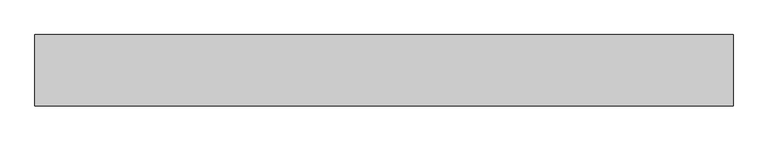
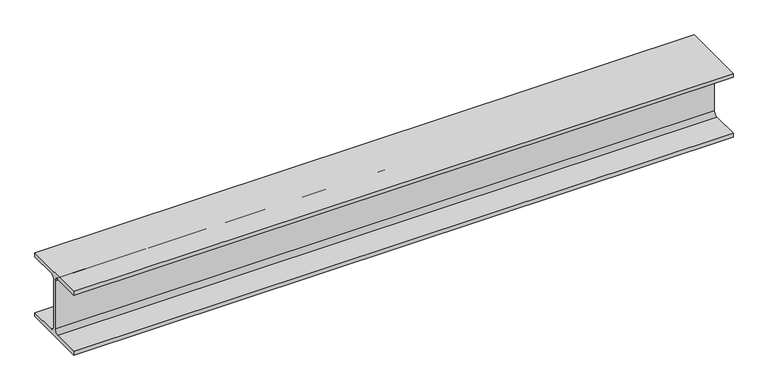
"""IFC4 building model written with IfcOpenShell, lengths in millimetres: beam geometry, 0912_Steel Framing_H-KSD3502 : H_SB_ASB_H-200x200x8x12."""

import ifcopenshell
import ifcopenshell.guid

model = None  # the IFC model being written
_history = None  # IfcOwnerHistory: only IFC2X3 demands one
_inside = {}  # id of a spatial element -> (the spatial element, [elements in it])
_under = {}  # id of a project, library or spatial element -> (it, [spatial elements below it])
_declared = {}  # id of a project -> (the project, [libraries it declares])
_typed = {}  # id of a type object -> (the type object, [elements of that type])
_made_of = {}  # id of a material, layer set ... -> (it, [elements and type objects made of it])


def new_model(schema):
    """Start an empty IFC model of exactly this schema.

    Asked for "IFC4X3", IfcOpenShell would pick the latest addendum, in which some entities
    have other attributes; the version numbers below select the first issue.
    IFC2X3 requires an IfcOwnerHistory on every rooted entity: one is made here for all.
    """
    global model, _history
    if schema == "IFC4X3":
        model = ifcopenshell.file(schema_version=(4, 3, 0, 0))
    else:
        model = ifcopenshell.file(schema=schema)
    _inside.clear()
    _under.clear()
    _declared.clear()
    _typed.clear()
    _made_of.clear()
    _history = None
    if model.schema == "IFC2X3":
        org = make("IfcOrganization", Name="unknown")
        user = make(
            "IfcPersonAndOrganization",
            ThePerson=make("IfcPerson", FamilyName="unknown"),
            TheOrganization=org,
        )
        app = make(
            "IfcApplication",
            ApplicationDeveloper=org,
            Version="unknown",
            ApplicationFullName="unknown",
            ApplicationIdentifier="unknown",
        )
        _history = make(
            "IfcOwnerHistory",
            OwningUser=user,
            OwningApplication=app,
            ChangeAction="ADDED",
            CreationDate=0,
        )
    return model


def make(cls, **values):
    """One entity of the class cls with the attributes given. An attribute that is None is left unset."""
    return model.create_entity(
        cls, **{name: value for name, value in values.items() if value is not None}
    )


def rooted(cls, **values):
    """An entity with a GlobalId (a new one), such as an element, a storey or a relation."""
    return make(cls, GlobalId=ifcopenshell.guid.new(), OwnerHistory=_history, **values)


def si_unit(unit_type, name, prefix=None):
    """IfcSIUnit, for example si_unit("LENGTHUNIT", "METRE", prefix="MILLI")."""
    return make("IfcSIUnit", UnitType=unit_type, Prefix=prefix, Name=name)


def assignment(units):
    """IfcUnitAssignment: the units of a project."""
    return None if units is None else make("IfcUnitAssignment", Units=units)


def point(xyz):
    """IfcCartesianPoint."""
    return None if xyz is None else make("IfcCartesianPoint", Coordinates=xyz)


def direction(xyz):
    """IfcDirection."""
    return None if xyz is None else make("IfcDirection", DirectionRatios=xyz)


def frame(location, z_axis=None, x_axis=None):
    """IfcAxis2Placement3D, a coordinate frame: its origin and axes. An axis left out is left unset."""
    return make(
        "IfcAxis2Placement3D",
        Location=point(location),
        Axis=direction(z_axis),
        RefDirection=direction(x_axis),
    )


def frame_2d(location, x_axis=None):
    """IfcAxis2Placement2D, a coordinate frame in the plane: its origin and x axis."""
    return make(
        "IfcAxis2Placement2D", Location=point(location), RefDirection=direction(x_axis)
    )


def origin():
    """The frame at (0, 0, 0) with its axes left unset."""
    return frame((0.0, 0.0, 0.0))


def place(relative_to, where):
    """IfcLocalPlacement: puts the frame where relative to a parent placement (None: the world)."""
    return make(
        "IfcLocalPlacement", PlacementRelTo=relative_to, RelativePlacement=where
    )


def context(
    kind, dimensions, precision=None, world=None, true_north=None, identifier=None
):
    """IfcGeometricRepresentationContext, for example the 3D "Model" context."""
    return make(
        "IfcGeometricRepresentationContext",
        ContextIdentifier=identifier,
        ContextType=kind,
        CoordinateSpaceDimension=dimensions,
        Precision=precision,
        WorldCoordinateSystem=world,
        TrueNorth=true_north,
    )


def project(units=None, contexts=None):
    """IfcProject with its units and contexts."""
    return rooted(
        "IfcProject",
        Name="project",
        RepresentationContexts=contexts,
        UnitsInContext=assignment(units),
    )


def spatial(cls, under=None, at=None, **own):
    """A site, building, storey or space (cls), placed at a placement, below another one or the project."""
    s = rooted(cls, ObjectPlacement=at, **own)
    if under is not None:
        _under.setdefault(under.id(), (under, []))[1].append(s)
    return s


def polyline(points):
    """IfcPolyline through the points."""
    return make("IfcPolyline", Points=[point(p) for p in points])


def circle_curve(where, radius):
    """IfcCircle in the frame where."""
    return make("IfcCircle", Position=where, Radius=radius)


def trimmed(basis, trim1, trim2, sense, master):
    """IfcTrimmedCurve: the piece of a basis curve between two trims."""
    return make(
        "IfcTrimmedCurve",
        BasisCurve=basis,
        Trim1=trim1,
        Trim2=trim2,
        SenseAgreement=sense,
        MasterRepresentation=master,
    )


def segment(curve, same_sense, transition):
    """IfcCompositeCurveSegment."""
    return make(
        "IfcCompositeCurveSegment",
        Transition=transition,
        SameSense=same_sense,
        ParentCurve=curve,
    )


def composite_curve(segments, self_intersect=None):
    """IfcCompositeCurve: segments joined end to end."""
    return make("IfcCompositeCurve", Segments=segments, SelfIntersect=self_intersect)


def outline(outer, holes=None, kind="AREA"):
    """IfcArbitraryClosedProfileDef: a profile drawn as a closed curve; with holes, ...WithVoids."""
    if holes is None:
        return make("IfcArbitraryClosedProfileDef", ProfileType=kind, OuterCurve=outer)
    return make(
        "IfcArbitraryProfileDefWithVoids",
        ProfileType=kind,
        OuterCurve=outer,
        InnerCurves=holes,
    )


def extrude(swept, where, along, depth):
    """IfcExtrudedAreaSolid: the profile swept, set in the frame where, extruded along a direction by depth."""
    return make(
        "IfcExtrudedAreaSolid",
        SweptArea=swept,
        Position=where,
        ExtrudedDirection=direction(along),
        Depth=depth,
    )


def shape(context_of_items, identifier, shape_type, items):
    """IfcShapeRepresentation: the items that make up one representation, for example the "Body"."""
    return make(
        "IfcShapeRepresentation",
        ContextOfItems=context_of_items,
        RepresentationIdentifier=identifier,
        RepresentationType=shape_type,
        Items=items,
    )


def source(mapping_origin, context_of_items, identifier, shape_type, items):
    """IfcRepresentationMap: a shape defined once, which mapped items show again and again."""
    return make(
        "IfcRepresentationMap",
        MappingOrigin=mapping_origin,
        MappedRepresentation=shape(context_of_items, identifier, shape_type, items),
    )


def transform(
    local_origin,
    x_axis=None,
    y_axis=None,
    z_axis=None,
    scale=None,
    scale2=None,
    scale3=None,
    uniform=True,
):
    """IfcCartesianTransformationOperator3D, or its non-uniform kind. x_axis, y_axis, z_axis: its Axis1, 2, 3."""
    if uniform:
        return make(
            "IfcCartesianTransformationOperator3D",
            Axis1=direction(x_axis),
            Axis2=direction(y_axis),
            LocalOrigin=point(local_origin),
            Scale=scale,
            Axis3=direction(z_axis),
        )
    return make(
        "IfcCartesianTransformationOperator3DnonUniform",
        Axis1=direction(x_axis),
        Axis2=direction(y_axis),
        LocalOrigin=point(local_origin),
        Scale=scale,
        Axis3=direction(z_axis),
        Scale2=scale2,
        Scale3=scale3,
    )


def mapped(mapping_source, mapping_target):
    """IfcMappedItem: shows the shape of a source again, moved by a transform."""
    return make(
        "IfcMappedItem", MappingSource=mapping_source, MappingTarget=mapping_target
    )


def made_of(thing, what):
    """Note that an element or type object is made of a material, layer set ...; save() writes the relation."""
    if what is not None:
        _made_of.setdefault(what.id(), (what, []))[1].append(thing)
    return thing


def element(
    cls,
    number,
    at=None,
    inside=None,
    cuts=None,
    type_object=None,
    material=None,
    context=None,
    identifier="Body",
    shape_type=None,
    held_by="IfcProductDefinitionShape",
    body=None,
    shapes=None,
    **own,
):
    """One element of the class cls, such as IfcWall. Its Tag is "e" and its number.

    at: its placement. inside: the storey or other place that contains it. cuts: it is an
    opening in that element (IfcRelVoidsElement). A single representation is given by context,
    identifier, shape_type and body (its items); several are given by shapes. held_by: the class
    of the entity that holds the representations. save() writes the other relations.
    """
    e = rooted(cls, Tag="e%d" % number, ObjectPlacement=at, **own)
    if body is not None:
        shapes = [shape(context, identifier, shape_type, body)]
    if shapes is not None:
        e.Representation = make(held_by, Representations=shapes)
    if inside is not None:
        _inside.setdefault(inside.id(), (inside, []))[1].append(e)
    if cuts is not None:
        rooted(
            "IfcRelVoidsElement", RelatingBuildingElement=cuts, RelatedOpeningElement=e
        )
    if type_object is not None:
        _typed.setdefault(type_object.id(), (type_object, []))[1].append(e)
    return made_of(e, material)


def aggregate(whole, parts):
    """IfcRelAggregates: a whole, such as a stair, and the parts it consists of."""
    return rooted("IfcRelAggregates", RelatingObject=whole, RelatedObjects=parts)


def save(model, path):
    """Write the relations noted so far, then the file.

    IfcRelAggregates (storeys below a building ...), IfcRelContainedInSpatialStructure (elements
    in a storey), IfcRelDefinesByType, IfcRelAssociatesMaterial and IfcRelDeclares: one each for
    every whole, place, type object, material and project.
    """
    for whole, parts in _under.values():
        aggregate(whole, parts)
    for where, things in _inside.values():
        rooted(
            "IfcRelContainedInSpatialStructure",
            RelatedElements=things,
            RelatingStructure=where,
        )
    for kind, things in _typed.values():
        rooted("IfcRelDefinesByType", RelatedObjects=things, RelatingType=kind)
    for what, things in _made_of.values():
        rooted("IfcRelAssociatesMaterial", RelatedObjects=things, RelatingMaterial=what)
    for by, libraries in _declared.values():
        rooted("IfcRelDeclares", RelatingContext=by, RelatedDefinitions=libraries)
    model.write(path)


def beam_1032c180(model_context):
    return source(origin(), model_context, "Body", "SweptSolid", [
        extrude(outline(composite_curve([segment(polyline([(100.0, -88.0), (100.0, -100.0), (-100.0, -100.0), (-100.0, -88.0), (-17.0, -88.0)]), True, "CONTINUOUS"), segment(trimmed(circle_curve(frame_2d((-17.0, -75.0)), 13.0), [point((-17.0, -88.0))], [point((-4.0, -75.0))], True, "CARTESIAN"), True, "CONTINUOUS"), segment(polyline([(-4.0, -75.0), (-4.0, 75.0)]), True, "CONTINUOUS"), segment(trimmed(circle_curve(frame_2d((-17.0, 75.0)), 13.0), [point((-4.0, 75.0))], [point((-17.0, 88.0))], True, "CARTESIAN"), True, "CONTINUOUS"), segment(polyline([(-17.0, 88.0), (-100.0, 88.0), (-100.0, 100.0), (100.0, 100.0), (100.0, 88.0), (17.0, 88.0)]), True, "CONTINUOUS"), segment(trimmed(circle_curve(frame_2d((17.0, 75.0)), 13.0), [point((17.0, 88.0))], [point((4.0, 75.0))], True, "CARTESIAN"), True, "CONTINUOUS"), segment(polyline([(4.0, 75.0), (4.0, -75.0)]), True, "CONTINUOUS"), segment(trimmed(circle_curve(frame_2d((17.0, -75.0)), 13.0), [point((4.0, -75.0))], [point((17.0, -88.0))], True, "CARTESIAN"), True, "CONTINUOUS"), segment(polyline([(17.0, -88.0), (100.0, -88.0)]), True, "CONTINUOUS")], self_intersect=False)), frame((-926.5182437, 0.0, 0.0), z_axis=(1.0, 0.0, 0.0), x_axis=(0.0, 1.0, 0.0)), (0.0, 0.0, 1.0), 1959.1715213),
    ])


if __name__ == "__main__":
    model = new_model("IFC4")
    model_context = context("Model", 3, world=origin())
    ifc_project = project(units=[si_unit("LENGTHUNIT", "METRE", prefix="MILLI")], contexts=[model_context])
    site = spatial("IfcSite", under=ifc_project)
    building = spatial("IfcBuilding", under=site)
    placement = place(None, origin())
    beam_shape = beam_1032c180(model_context)
    element("IfcBeam", 1, ObjectType="0912_Steel Framing_H-KSD3502 : H_SB_ASB_H-200x200x8x12", at=placement, inside=building, context=model_context, shape_type="MappedRepresentation", body=[
        mapped(beam_shape, transform((0.0, 0.0, 0.0), x_axis=(1.0, 0.0, 0.0), y_axis=(0.0, 1.0, 0.0), z_axis=(0.0, 0.0, 1.0))),
    ])
    save(model, "model.ifc")

# Revit data of these elements
# Type "0912_Steel Framing_H-KSD3502 : H_SB_ASB_H-200x200x8x12"
#   H_WM Code_1 = "S01AA002-00001 | Main Steel Structure Fabrication Work | Shelter/Building | Medium Steel - Standard (90KG/M>Weight≥30KG/M) | Material: (   )"
#   H_WM Code_2 = "S03AA028-00001 | Main Steel Structure Erection Work | Shelter/Building | Medium Steel (90KG/M>Weight≥30KG/M) | Material: (   )"
#   H_WM Code_3 = "S01AA010-00001 | Main Steel Structure Fabrication Work | Shelter/Building | Steel Painting/Coating | for Non-Fireproofed Steel Surface, Surface Preparation, Primer, Second & Final Coat | Material: (   )"
#   H_Q'ty Cal Type Tag = "SB-Q2"
#   Width = 20.0 cm
#   Web Thickness = 0.8 cm
#   Web Fillet = 1.3 cm
#   Warping Constant = 141000.0 cm⁶
#   W = 0
#   Torsional Moment of Inertia = 26.2485 cm⁴
#   Section Area = 63.53 cm²
#   Plastic Modulus weak axis = 244.0 cm³
#   Plastic Modulus strong axis = 525.0 cm³
#   Perimeter = 1.16 m²/m
#   Nominal Weight = 49.90 kgf/m
#   Moment of Inertia weak axis = 1600.00 cm⁴
#   Moment of Inertia strong axis = 4720.00 cm⁴
#   Height = 20.0 cm
#   Flange Thickness = 1.2 cm
#   Elastic Modulus weak axis = 160.0 cm³
#   Elastic Modulus strong axis = 472.0 cm³
#   Centroid Vertical = 10.0 cm
#   Centroid Horizontal = 10.0 cm
#   Ix = 47200000
#   Length [instance default] = 1.5240 m
#   Zx = 525000
#   b = 0.2000 m
#   h = 0.2000 m
#   r = 0.0130 m
#   s = 0.0080 m
#   t = 0.0120 m
#   A = 0.006353 m²
#   Structural Material [instance default] = Steel, 45-345
#   Assembly Code = ""
# Element 1 (IfcBeam, "0912_Steel Framing_H-KSD3502 : H_SB_ASB_H-200x200x8x12")
#   Structural Material = none
# Materials
#   "Steel, 45-345": class "Metal", colour RGB 189 187 185, transparency 0, Description = "Steel 345 MPa", Cost = 0
